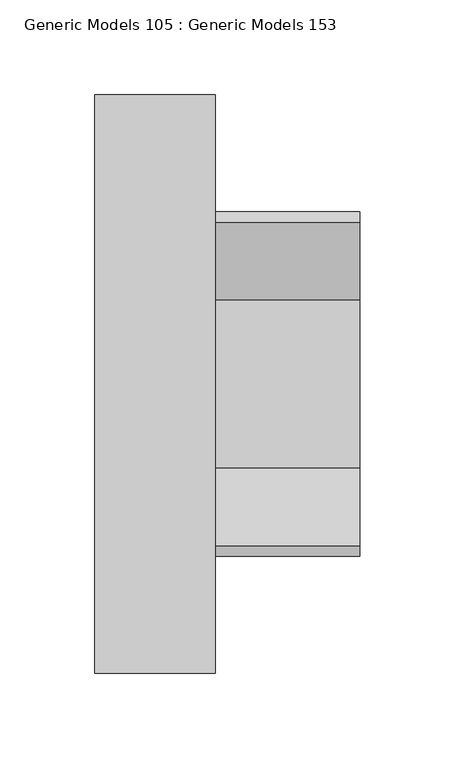
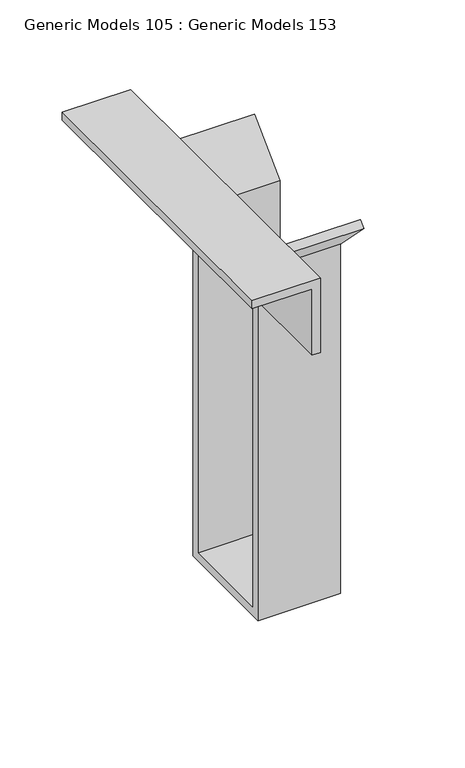
"""IFC4 building model written with IfcOpenShell, lengths in millimetres: proxy geometry, Generic Models 105 : Generic Models 153."""

from ifc_helpers import new_model, si_unit, frame, origin, place, context, project, spatial, polyline, outline, extrude, source, transform, mapped, element, save


def generic_models_105_generic_models_153_b6c06995(model_context):
    return source(origin(), model_context, "Body", "SweptSolid", [
        extrude(outline(polyline([(35194.5707942, 269095.5375), (35194.5707942, 268757.4), (35283.4707942, 268757.4), (35283.4707942, 269095.5375), (35324.2643041, 269136.3310099), (35329.8769642, 269130.7183498), (35291.4082942, 269092.2496798), (35291.4082942, 268749.4625), (35186.6332942, 268749.4625), (35186.6332942, 269092.2496798), (35148.1646242, 269130.7183498), (35153.7772843, 269136.3310099), (35194.5707942, 269095.5375)])), frame((32208.7960525, 0.0, 0.0), z_axis=(1.0, 0.0, 0.0), x_axis=(0.0, 1.0, 0.0)), (0.0, 0.0, 1.0), 76.2),
        extrude(outline(polyline([(269138.4, 32145.2960525), (269138.4, 32200.8585525), (269073.3125, 32200.8585525), (269073.3125, 32208.7960525), (269146.3375, 32208.7960525), (269146.3375, 32145.2960525), (269138.4, 32145.2960525)])), frame((0.0, 35086.6207942, 0.0), z_axis=(0.0, 1.0, 0.0), x_axis=(0.0, 0.0, 1.0)), (0.0, 0.0, 1.0), 304.8),
    ])


if __name__ == "__main__":
    model = new_model("IFC4")
    model_context = context("Model", 3, world=origin())
    ifc_project = project(units=[si_unit("LENGTHUNIT", "METRE", prefix="MILLI")], contexts=[model_context])
    site = spatial("IfcSite", under=ifc_project)
    building = spatial("IfcBuilding", under=site)
    placement = place(None, origin())
    generic_models_105_generic_models_153_shape = generic_models_105_generic_models_153_b6c06995(model_context)
    element("IfcBuildingElementProxy", 1, Name="Generic Models 105 : Generic Models 153", ObjectType="Generic Models 105 : Generic Models 153", at=placement, inside=building, context=model_context, shape_type="MappedRepresentation", body=[
        mapped(generic_models_105_generic_models_153_shape, transform((0.0, 0.0, 0.0), x_axis=(1.0, 0.0, 0.0), y_axis=(0.0, 1.0, 0.0), z_axis=(0.0, 0.0, 1.0))),
    ])
    save(model, "model.ifc")

# Revit data of these elements
# Element 1 (IfcBuildingElementProxy, "Generic Models 105 : Generic Models 153")
#   Materials on its faces: "SIMPSON GLT HANGER (GALVANIZED)"
# Materials
#   "SIMPSON GLT HANGER (GALVANIZED)": class "Metal", colour RGB 199 199 199, transparency 0, Description = "Carbon steel", Cost = 0
